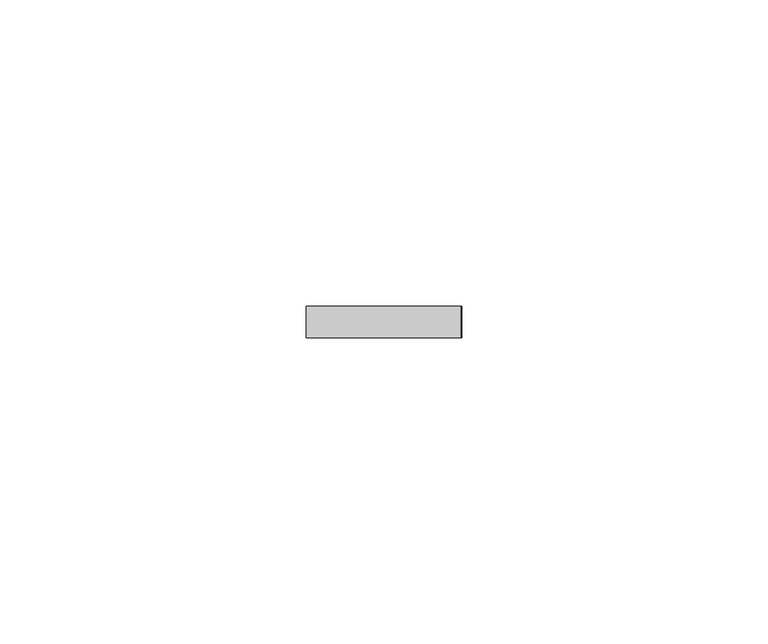
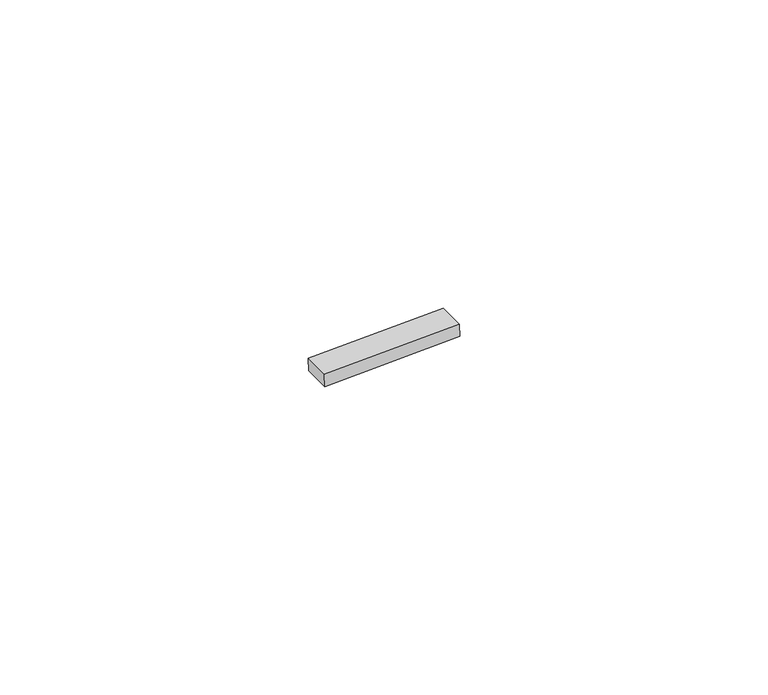
"""IFC4 building model written with IfcOpenShell, lengths in millimetres: proxy geometry, Inner panel:Inner panel:1:Inner panel:1 : Inner panel:Inner panel:300324:2:Inner panel:1:Inner panel:1 : Inner panel:Inner panel:300324:2 : Inner panel:Inner panel:1:Inner panel:1 : Inner panel:Inner panel:300324:300043:175 : Inner panel:Inner panel:1:Inner panel:1 : Inner panel:Inner panel:300324:2:Inner panel:1:Inner panel:1 : Inner panel:Inner panel:300324:2 : Inner panel:Inner panel:1:Inner panel:1 : Inner panel:Inner panel:300324:300043:308120."""

from ifc_helpers import new_model, si_unit, frame, origin, place, context, project, spatial, polyline, outline, extrude, source, transform, mapped, element, save


def generic_models_9a78f3c5(model_context):
    return source(origin(), model_context, "Body", "SweptSolid", [
        extrude(outline(polyline([(0.0, -25.4), (0.0, 0.0), (5.213809, 0.0), (5.213809, -25.4), (0.0, -25.4)])), frame((560380.9331581, -566213.307991, 3950.5346612), z_axis=(-0.041630544712223896, 0.0, 0.9991330730923502), x_axis=(0.0, -1.0, 0.0)), (0.0, 0.0, 1.0), 2.4763745),
    ])


if __name__ == "__main__":
    model = new_model("IFC4")
    model_context = context("Model", 3, world=origin())
    ifc_project = project(units=[si_unit("LENGTHUNIT", "METRE", prefix="MILLI")], contexts=[model_context])
    site = spatial("IfcSite", under=ifc_project)
    building = spatial("IfcBuilding", under=site)
    placement = place(None, origin())
    generic_models_shape = generic_models_9a78f3c5(model_context)
    element("IfcBuildingElementProxy", 1, Name="Inner panel:Inner panel:1:Inner panel:1 : Inner panel:Inner panel:300324:2:Inner panel:1:Inner panel:1 : Inner panel:Inner panel:300324:2 : Inner panel:Inner panel:1:Inner panel:1 : Inner panel:Inner panel:300324:300043:175 : Inner panel:Inner panel:1:Inner panel:1 : Inner panel:Inner panel:300324:2:Inner panel:1:Inner panel:1 : Inner panel:Inner panel:300324:2 : Inner panel:Inner panel:1:Inner panel:1 : Inner panel:Inner panel:300324:300043:308120", ObjectType="Inner panel:Inner panel:1:Inner panel:1 : Inner panel:Inner panel:300324:2:Inner panel:1:Inner panel:1 : Inner panel:Inner panel:300324:2 : Inner panel:Inner panel:1:Inner panel:1 : Inner panel:Inner panel:300324:300043:175 : Inner panel:Inner panel:1:Inner panel:1 : Inner panel:Inner panel:300324:2:Inner panel:1:Inner panel:1 : Inner panel:Inner panel:300324:2 : Inner panel:Inner panel:1:Inner panel:1 : Inner panel:Inner panel:300324:300043:308120", at=placement, inside=building, context=model_context, shape_type="MappedRepresentation", body=[
        mapped(generic_models_shape, transform((0.0, 0.0, 0.0), x_axis=(1.0, 0.0, 0.0), y_axis=(0.0, 1.0, 0.0), z_axis=(0.0, 0.0, 1.0))),
    ])
    save(model, "model.ifc")

# Revit data of these elements
# Type "Inner panel:Inner panel:1:Inner panel:1 : Inner panel:Inner panel:300324:2:Inner panel:1:Inner panel:1 : Inner panel:Inner panel:300324:2 : Inner panel:Inner panel:1:Inner panel:1 : Inner panel:Inner panel:300324:300043:175 : Inner panel:Inner panel:1:Inner panel:1 : Inner panel:Inner panel:300324:2:Inner panel:1:Inner panel:1 : Inner panel:Inner panel:300324:2 : Inner panel:Inner panel:1:Inner panel:1 : Inner panel:Inner panel:300324:300043:308120"
#   NameOverride = "Inner panel:Inner panel:1:Inner panel:1 : Inner panel:Inner panel:300324:2:Inner panel:1:Inner panel:1 : Inner panel:Inner panel:300324:2 : Inner panel:Inner panel:1:Inner panel:1 : Inner panel:Inner panel:300324:300043:308120"
#   ObjectTypeOverride = "Inner panel:1:Inner panel:1 : Inner panel:Inner panel:300324:2 : Inner panel:Inner panel:1:Inner panel:1 : Inner panel:Inner panel:300324:300043"
#   Reference = "Inner panel"
#   Tag = "308120"
# Element 1 (IfcBuildingElementProxy, "Inner panel:Inner panel:1:Inner panel:1 : Inner panel:Inner panel:300324:2:Inner panel:1:Inner panel:1 : Inner panel:Inner panel:300324:2 : Inner panel:Inner panel:1:Inner panel:1 : Inner panel:Inner panel:300324:300043:175 : Inner panel:Inner panel:1:Inner panel:1 : Inner panel:Inner panel:300324:2:Inner panel:1:Inner panel:1 : Inner panel:Inner panel:300324:2 : Inner panel:Inner panel:1:Inner panel:1 : Inner panel:Inner panel:300324:300043:308120")
#   Materials on its faces: "AT CLIP - 1\" WIDE NON ABSORBENT, WEATHER-RESISTANT NEOPRENE/EPDM/SBR FOAM"
# Materials
#   "AT CLIP - 1\" WIDE NON ABSORBENT, WEATHER-RESISTANT NEOPRENE/EPDM/SBR FOAM": class "Generic", colour RGB 85 85 85, transparency 0, Cost = 0
